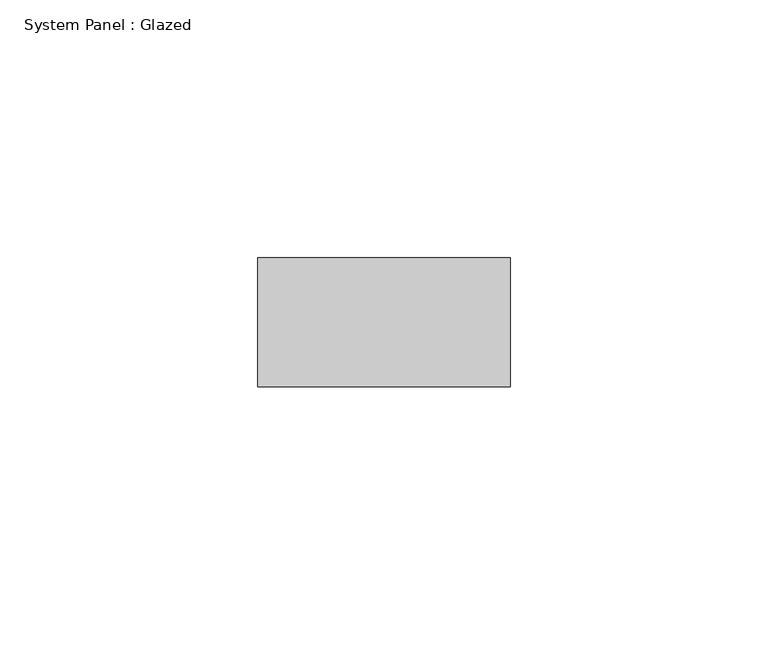
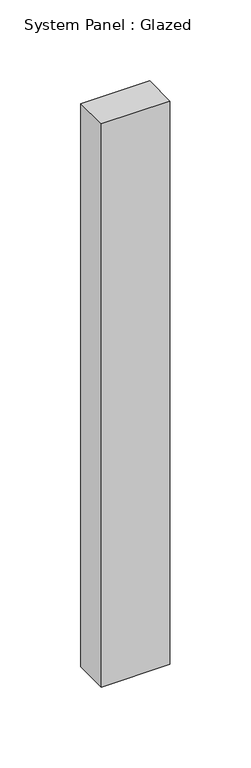
"""IFC4 building model written with IfcOpenShell, lengths in millimetres: plate geometry, System Panel : Glazed."""

from ifc_helpers import new_model, si_unit, origin, origin_with_axes, place, context, project, spatial, polyline, outline, extrude, source, transform, mapped, element, save


def system_panel_glazed_0535c902(model_context):
    return source(origin(), model_context, "Body", "SweptSolid", [
        extrude(outline(polyline([(24.5092572, -49.5), (-24.5092572, -49.5), (-24.5092572, -24.5), (24.5092572, -24.5), (24.5092572, -49.5)])), origin_with_axes(), (0.0, 0.0, 1.0), 425.0),
    ])


if __name__ == "__main__":
    model = new_model("IFC4")
    model_context = context("Model", 3, world=origin())
    ifc_project = project(units=[si_unit("LENGTHUNIT", "METRE", prefix="MILLI")], contexts=[model_context])
    site = spatial("IfcSite", under=ifc_project)
    building = spatial("IfcBuilding", under=site)
    placement = place(None, origin())
    system_panel_glazed_shape = system_panel_glazed_0535c902(model_context)
    element("IfcPlate", 1, ObjectType="System Panel : Glazed", at=placement, inside=building, context=model_context, shape_type="MappedRepresentation", body=[
        mapped(system_panel_glazed_shape, transform((0.0, 0.0, 0.0), x_axis=(1.0, 0.0, 0.0), y_axis=(0.0, 1.0, 0.0), z_axis=(0.0, 0.0, 1.0))),
    ])
    save(model, "model.ifc")

# Revit data of these elements
# Project information
#   Project Issue Date = "Issue Date"
#   Project Status = "Project Status"
#   Project Address = "Enter address here"
#   Project Name = "MASS BUILDING"
#   Project Number = "Project Number"
# Type "System Panel : Glazed"
#   Keynote = "H11"
#   Construction Type Id = "GSP4R"
#   Analytic Construction = "1/8 in Pilkington single glazing"
#   Visual Light Transmittance = 0.9
#   Solar Heat Gain Coefficient = 0.86
#   Heat Transfer Coefficient (U) = 6.7069 W/(m²·K)
# Element 1 (IfcPlate, "System Panel : Glazed")
#   Materials on its faces: "Glass"
# Materials
#   "Glass": class "Glass", colour RGB 0 128 192, transparency 0.9, Description = "Soda Lime Glass", Cost = 0
